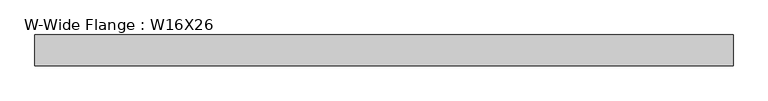
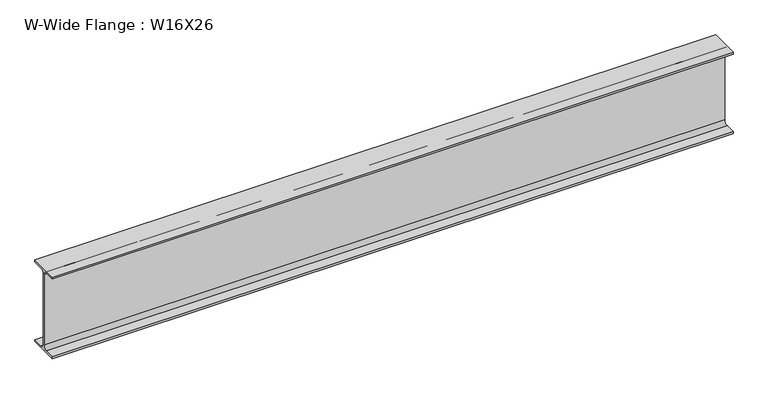
"""IFC4 building model written with IfcOpenShell, lengths in millimetres: beam geometry, W-Wide Flange : W16X26."""

import ifcopenshell
import ifcopenshell.guid

model = None  # the IFC model being written
_history = None  # IfcOwnerHistory: only IFC2X3 demands one
_inside = {}  # id of a spatial element -> (the spatial element, [elements in it])
_under = {}  # id of a project, library or spatial element -> (it, [spatial elements below it])
_declared = {}  # id of a project -> (the project, [libraries it declares])
_typed = {}  # id of a type object -> (the type object, [elements of that type])
_made_of = {}  # id of a material, layer set ... -> (it, [elements and type objects made of it])


def new_model(schema):
    """Start an empty IFC model of exactly this schema.

    Asked for "IFC4X3", IfcOpenShell would pick the latest addendum, in which some entities
    have other attributes; the version numbers below select the first issue.
    IFC2X3 requires an IfcOwnerHistory on every rooted entity: one is made here for all.
    """
    global model, _history
    if schema == "IFC4X3":
        model = ifcopenshell.file(schema_version=(4, 3, 0, 0))
    else:
        model = ifcopenshell.file(schema=schema)
    _inside.clear()
    _under.clear()
    _declared.clear()
    _typed.clear()
    _made_of.clear()
    _history = None
    if model.schema == "IFC2X3":
        org = make("IfcOrganization", Name="unknown")
        user = make(
            "IfcPersonAndOrganization",
            ThePerson=make("IfcPerson", FamilyName="unknown"),
            TheOrganization=org,
        )
        app = make(
            "IfcApplication",
            ApplicationDeveloper=org,
            Version="unknown",
            ApplicationFullName="unknown",
            ApplicationIdentifier="unknown",
        )
        _history = make(
            "IfcOwnerHistory",
            OwningUser=user,
            OwningApplication=app,
            ChangeAction="ADDED",
            CreationDate=0,
        )
    return model


def make(cls, **values):
    """One entity of the class cls with the attributes given. An attribute that is None is left unset."""
    return model.create_entity(
        cls, **{name: value for name, value in values.items() if value is not None}
    )


def rooted(cls, **values):
    """An entity with a GlobalId (a new one), such as an element, a storey or a relation."""
    return make(cls, GlobalId=ifcopenshell.guid.new(), OwnerHistory=_history, **values)


def si_unit(unit_type, name, prefix=None):
    """IfcSIUnit, for example si_unit("LENGTHUNIT", "METRE", prefix="MILLI")."""
    return make("IfcSIUnit", UnitType=unit_type, Prefix=prefix, Name=name)


def assignment(units):
    """IfcUnitAssignment: the units of a project."""
    return None if units is None else make("IfcUnitAssignment", Units=units)


def point(xyz):
    """IfcCartesianPoint."""
    return None if xyz is None else make("IfcCartesianPoint", Coordinates=xyz)


def direction(xyz):
    """IfcDirection."""
    return None if xyz is None else make("IfcDirection", DirectionRatios=xyz)


def frame(location, z_axis=None, x_axis=None):
    """IfcAxis2Placement3D, a coordinate frame: its origin and axes. An axis left out is left unset."""
    return make(
        "IfcAxis2Placement3D",
        Location=point(location),
        Axis=direction(z_axis),
        RefDirection=direction(x_axis),
    )


def frame_2d(location, x_axis=None):
    """IfcAxis2Placement2D, a coordinate frame in the plane: its origin and x axis."""
    return make(
        "IfcAxis2Placement2D", Location=point(location), RefDirection=direction(x_axis)
    )


def origin():
    """The frame at (0, 0, 0) with its axes left unset."""
    return frame((0.0, 0.0, 0.0))


def place(relative_to, where):
    """IfcLocalPlacement: puts the frame where relative to a parent placement (None: the world)."""
    return make(
        "IfcLocalPlacement", PlacementRelTo=relative_to, RelativePlacement=where
    )


def context(
    kind, dimensions, precision=None, world=None, true_north=None, identifier=None
):
    """IfcGeometricRepresentationContext, for example the 3D "Model" context."""
    return make(
        "IfcGeometricRepresentationContext",
        ContextIdentifier=identifier,
        ContextType=kind,
        CoordinateSpaceDimension=dimensions,
        Precision=precision,
        WorldCoordinateSystem=world,
        TrueNorth=true_north,
    )


def project(units=None, contexts=None):
    """IfcProject with its units and contexts."""
    return rooted(
        "IfcProject",
        Name="project",
        RepresentationContexts=contexts,
        UnitsInContext=assignment(units),
    )


def spatial(cls, under=None, at=None, **own):
    """A site, building, storey or space (cls), placed at a placement, below another one or the project."""
    s = rooted(cls, ObjectPlacement=at, **own)
    if under is not None:
        _under.setdefault(under.id(), (under, []))[1].append(s)
    return s


def polyline(points):
    """IfcPolyline through the points."""
    return make("IfcPolyline", Points=[point(p) for p in points])


def circle_curve(where, radius):
    """IfcCircle in the frame where."""
    return make("IfcCircle", Position=where, Radius=radius)


def trimmed(basis, trim1, trim2, sense, master):
    """IfcTrimmedCurve: the piece of a basis curve between two trims."""
    return make(
        "IfcTrimmedCurve",
        BasisCurve=basis,
        Trim1=trim1,
        Trim2=trim2,
        SenseAgreement=sense,
        MasterRepresentation=master,
    )


def segment(curve, same_sense, transition):
    """IfcCompositeCurveSegment."""
    return make(
        "IfcCompositeCurveSegment",
        Transition=transition,
        SameSense=same_sense,
        ParentCurve=curve,
    )


def composite_curve(segments, self_intersect=None):
    """IfcCompositeCurve: segments joined end to end."""
    return make("IfcCompositeCurve", Segments=segments, SelfIntersect=self_intersect)


def outline(outer, holes=None, kind="AREA"):
    """IfcArbitraryClosedProfileDef: a profile drawn as a closed curve; with holes, ...WithVoids."""
    if holes is None:
        return make("IfcArbitraryClosedProfileDef", ProfileType=kind, OuterCurve=outer)
    return make(
        "IfcArbitraryProfileDefWithVoids",
        ProfileType=kind,
        OuterCurve=outer,
        InnerCurves=holes,
    )


def extrude(swept, where, along, depth):
    """IfcExtrudedAreaSolid: the profile swept, set in the frame where, extruded along a direction by depth."""
    return make(
        "IfcExtrudedAreaSolid",
        SweptArea=swept,
        Position=where,
        ExtrudedDirection=direction(along),
        Depth=depth,
    )


def shape(context_of_items, identifier, shape_type, items):
    """IfcShapeRepresentation: the items that make up one representation, for example the "Body"."""
    return make(
        "IfcShapeRepresentation",
        ContextOfItems=context_of_items,
        RepresentationIdentifier=identifier,
        RepresentationType=shape_type,
        Items=items,
    )


def source(mapping_origin, context_of_items, identifier, shape_type, items):
    """IfcRepresentationMap: a shape defined once, which mapped items show again and again."""
    return make(
        "IfcRepresentationMap",
        MappingOrigin=mapping_origin,
        MappedRepresentation=shape(context_of_items, identifier, shape_type, items),
    )


def transform(
    local_origin,
    x_axis=None,
    y_axis=None,
    z_axis=None,
    scale=None,
    scale2=None,
    scale3=None,
    uniform=True,
):
    """IfcCartesianTransformationOperator3D, or its non-uniform kind. x_axis, y_axis, z_axis: its Axis1, 2, 3."""
    if uniform:
        return make(
            "IfcCartesianTransformationOperator3D",
            Axis1=direction(x_axis),
            Axis2=direction(y_axis),
            LocalOrigin=point(local_origin),
            Scale=scale,
            Axis3=direction(z_axis),
        )
    return make(
        "IfcCartesianTransformationOperator3DnonUniform",
        Axis1=direction(x_axis),
        Axis2=direction(y_axis),
        LocalOrigin=point(local_origin),
        Scale=scale,
        Axis3=direction(z_axis),
        Scale2=scale2,
        Scale3=scale3,
    )


def mapped(mapping_source, mapping_target):
    """IfcMappedItem: shows the shape of a source again, moved by a transform."""
    return make(
        "IfcMappedItem", MappingSource=mapping_source, MappingTarget=mapping_target
    )


def made_of(thing, what):
    """Note that an element or type object is made of a material, layer set ...; save() writes the relation."""
    if what is not None:
        _made_of.setdefault(what.id(), (what, []))[1].append(thing)
    return thing


def element(
    cls,
    number,
    at=None,
    inside=None,
    cuts=None,
    type_object=None,
    material=None,
    context=None,
    identifier="Body",
    shape_type=None,
    held_by="IfcProductDefinitionShape",
    body=None,
    shapes=None,
    **own,
):
    """One element of the class cls, such as IfcWall. Its Tag is "e" and its number.

    at: its placement. inside: the storey or other place that contains it. cuts: it is an
    opening in that element (IfcRelVoidsElement). A single representation is given by context,
    identifier, shape_type and body (its items); several are given by shapes. held_by: the class
    of the entity that holds the representations. save() writes the other relations.
    """
    e = rooted(cls, Tag="e%d" % number, ObjectPlacement=at, **own)
    if body is not None:
        shapes = [shape(context, identifier, shape_type, body)]
    if shapes is not None:
        e.Representation = make(held_by, Representations=shapes)
    if inside is not None:
        _inside.setdefault(inside.id(), (inside, []))[1].append(e)
    if cuts is not None:
        rooted(
            "IfcRelVoidsElement", RelatingBuildingElement=cuts, RelatedOpeningElement=e
        )
    if type_object is not None:
        _typed.setdefault(type_object.id(), (type_object, []))[1].append(e)
    return made_of(e, material)


def aggregate(whole, parts):
    """IfcRelAggregates: a whole, such as a stair, and the parts it consists of."""
    return rooted("IfcRelAggregates", RelatingObject=whole, RelatedObjects=parts)


def save(model, path):
    """Write the relations noted so far, then the file.

    IfcRelAggregates (storeys below a building ...), IfcRelContainedInSpatialStructure (elements
    in a storey), IfcRelDefinesByType, IfcRelAssociatesMaterial and IfcRelDeclares: one each for
    every whole, place, type object, material and project.
    """
    for whole, parts in _under.values():
        aggregate(whole, parts)
    for where, things in _inside.values():
        rooted(
            "IfcRelContainedInSpatialStructure",
            RelatedElements=things,
            RelatingStructure=where,
        )
    for kind, things in _typed.values():
        rooted("IfcRelDefinesByType", RelatedObjects=things, RelatingType=kind)
    for what, things in _made_of.values():
        rooted("IfcRelAssociatesMaterial", RelatedObjects=things, RelatingMaterial=what)
    for by, libraries in _declared.values():
        rooted("IfcRelDeclares", RelatingContext=by, RelatedDefinitions=libraries)
    model.write(path)


def w_wide_flange_w16x26_461747bc(model_context):
    return source(origin(), model_context, "Body", "SweptSolid", [
        extrude(outline(composite_curve([segment(polyline([(69.85, -190.627), (69.85, -199.39), (-69.85, -199.39), (-69.85, -190.627), (-21.3995, -190.627)]), True, "CONTINUOUS"), segment(trimmed(circle_curve(frame_2d((-21.3995, -172.4025)), 18.2245), [point((-21.3995, -190.627))], [point((-3.175, -172.4025))], True, "CARTESIAN"), True, "CONTINUOUS"), segment(polyline([(-3.175, -172.4025), (-3.175, 172.4025)]), True, "CONTINUOUS"), segment(trimmed(circle_curve(frame_2d((-21.3995, 172.4025)), 18.2245), [point((-3.175, 172.4025))], [point((-21.3995, 190.627))], True, "CARTESIAN"), True, "CONTINUOUS"), segment(polyline([(-21.3995, 190.627), (-69.85, 190.627), (-69.85, 199.39), (69.85, 199.39), (69.85, 190.627), (21.3995, 190.627)]), True, "CONTINUOUS"), segment(trimmed(circle_curve(frame_2d((21.3995, 172.4025)), 18.2245), [point((21.3995, 190.627))], [point((3.175, 172.4025))], True, "CARTESIAN"), True, "CONTINUOUS"), segment(polyline([(3.175, 172.4025), (3.175, -172.4025)]), True, "CONTINUOUS"), segment(trimmed(circle_curve(frame_2d((21.3995, -172.4025)), 18.2245), [point((3.175, -172.4025))], [point((21.3995, -190.627))], True, "CARTESIAN"), True, "CONTINUOUS"), segment(polyline([(21.3995, -190.627), (69.85, -190.627)]), True, "CONTINUOUS")], self_intersect=False)), frame((-1574.8, 0.0, 0.0), z_axis=(1.0, 0.0, 0.0), x_axis=(0.0, 1.0, 0.0)), (0.0, 0.0, 1.0), 3149.6),
    ])


if __name__ == "__main__":
    model = new_model("IFC4")
    model_context = context("Model", 3, world=origin())
    ifc_project = project(units=[si_unit("LENGTHUNIT", "METRE", prefix="MILLI")], contexts=[model_context])
    site = spatial("IfcSite", under=ifc_project)
    building = spatial("IfcBuilding", under=site)
    placement = place(None, origin())
    w_wide_flange_w16x26_shape = w_wide_flange_w16x26_461747bc(model_context)
    element("IfcBeam", 1, ObjectType="W-Wide Flange : W16X26", at=placement, inside=building, context=model_context, shape_type="MappedRepresentation", body=[
        mapped(w_wide_flange_w16x26_shape, transform((0.0, 0.0, 0.0), x_axis=(1.0, 0.0, 0.0), y_axis=(0.0, 1.0, 0.0), z_axis=(0.0, 0.0, 1.0))),
    ])
    save(model, "model.ifc")

# Revit data of these elements
# Type "W-Wide Flange : W16X26"
#   Assembly Code = "B10"
#   W = 26
#   Length [instance default] = 5' - 0"
#   bf = 0' - 5 1/2"
#   d = 1' - 3.7"
#   k = 0' - 1 1/16"
#   k2 = 0' - 0.7175"
#   tf = 0' - 0.345"
#   tw = 0' - 0 1/4"
#   A = 0.0533333 SF
#   Structural Material [instance default] = Steel ASTM A992
# Element 1 (IfcBeam, "W-Wide Flange : W16X26")
#   Materials on its faces: "Steel ASTM A992"
# Materials
#   "Steel ASTM A992": class "Metal", colour RGB 199 199 199, transparency 0, Description = "Structural steel 50ksi", Cost = 0
